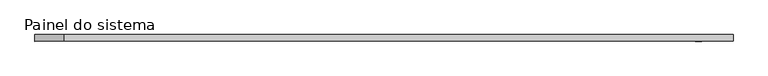
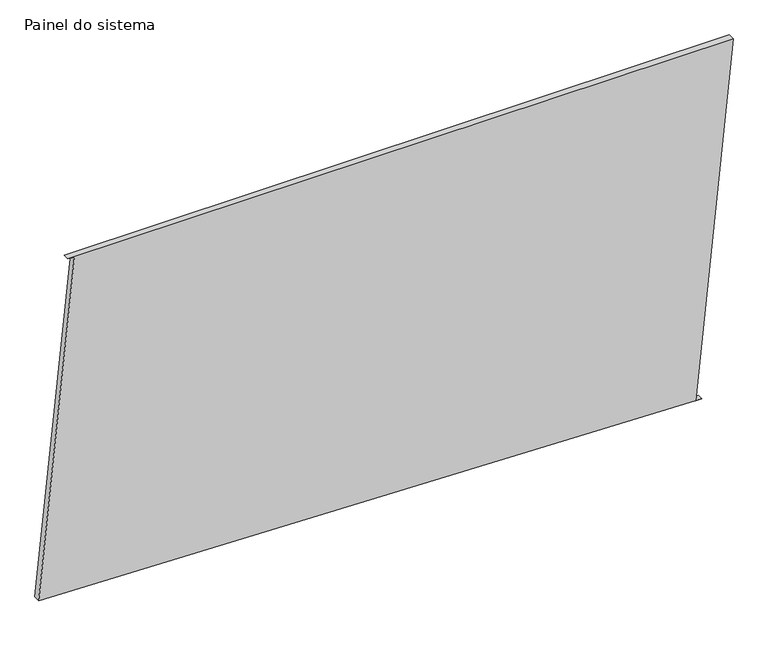
"""IFC4 building model written with IfcOpenShell, lengths in millimetres: plate geometry, Painel do sistema : Envidraçado."""

from ifc_helpers import new_model, si_unit, frame, origin, place, context, project, spatial, polyline, outline, extrude, source, transform, mapped, element, save


def painel_do_sistema_609f1617(model_context):
    return source(origin(), model_context, "Body", "SweptSolid", [
        extrude(outline(polyline([(0.0, 1216.7684439), (2.5300763, 1191.8967991), (1424.6077437, 1336.5581205), (1424.6077437, -1224.2183792), (1422.0776675, -1199.3467344), (73.2357927, -1336.5581205), (0.0, 1216.7684439)])), frame((0.0, 24.5, 0.0), z_axis=(0.0, 1.0, 0.0), x_axis=(0.0, 0.0, 1.0)), (0.0, 0.0, 1.0), 25.0),
    ])


if __name__ == "__main__":
    model = new_model("IFC4")
    model_context = context("Model", 3, world=origin())
    ifc_project = project(units=[si_unit("LENGTHUNIT", "METRE", prefix="MILLI")], contexts=[model_context])
    site = spatial("IfcSite", under=ifc_project)
    building = spatial("IfcBuilding", under=site)
    placement = place(None, origin())
    painel_do_sistema_shape = painel_do_sistema_609f1617(model_context)
    element("IfcPlate", 1, ObjectType="Painel do sistema : Envidraçado", at=placement, inside=building, context=model_context, shape_type="MappedRepresentation", body=[
        mapped(painel_do_sistema_shape, transform((0.0, 0.0, 0.0), x_axis=(1.0, 0.0, 0.0), y_axis=(0.0, 1.0, 0.0), z_axis=(0.0, 0.0, 1.0))),
    ])
    save(model, "model.ifc")

# Revit data of these elements
# Type "Painel do sistema : Envidraçado"
#   Construction Type Id = "GSP4R"
#   Analytic Construction = "Vidraça única Pilkington 1/8 pol"
#   Visual Light Transmittance = 0.9
#   Solar Heat Gain Coefficient = 0.86
#   Heat Transfer Coefficient (U) = 6.7069 W/(m²·K)
# Element 1 (IfcPlate, "Painel do sistema : Envidraçado")
#   Materials on its faces: "Vidro"
# Materials
#   "Vidro": class "Vidro", colour RGB 0 128 192, transparency 0.9, Description = "Vidro de sílica", Cost = 0
